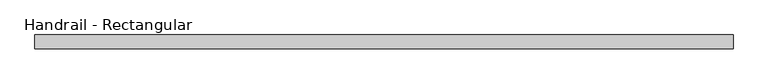
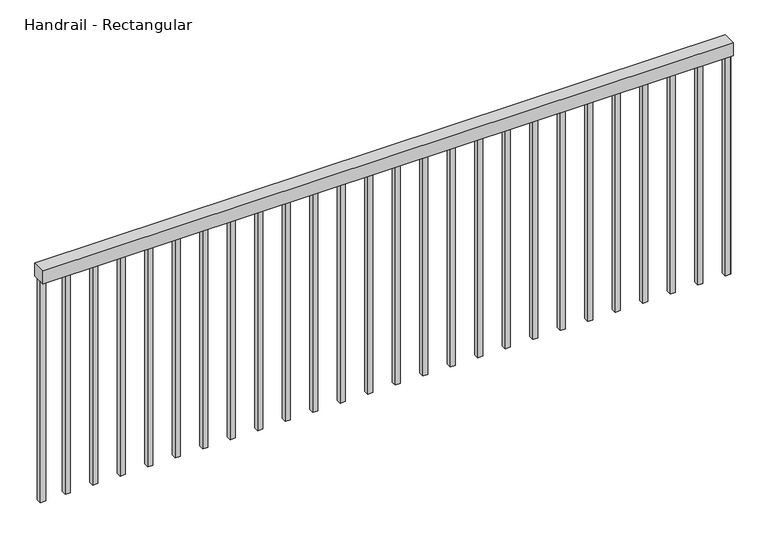
"""IFC4 building model written with IfcOpenShell, lengths in millimetres: railing geometry, Handrail - Rectangular."""

from ifc_helpers import new_model, si_unit, frame, origin, place, context, project, spatial, polyline, outline, extrude, source, transform, mapped, element, save


def handrail_rectangular_395b2247(model_context):
    return source(origin(), model_context, "Body", "SweptSolid", [
        extrude(outline(polyline([(-10635.2211091, 12195.0507146), (-10635.2211091, 12245.8507146), (-8085.2211091, 12245.8507146), (-8085.2211091, 12195.0507146), (-10635.2211091, 12195.0507146)])), frame((0.0, 0.0, 6654.4), z_axis=(0.0, 0.0, 1.0), x_axis=(1.0, 0.0, 0.0)), (0.0, 0.0, 1.0), 50.8),
        extrude(outline(polyline([(-8104.7461091, 12210.9257146), (-8104.7461091, 12229.9757146), (-8085.6961091, 12229.9757146), (-8085.6961091, 12210.9257146), (-8104.7461091, 12210.9257146)])), frame((0.0, 0.0, 5790.8), z_axis=(0.0, 0.0, 1.0), x_axis=(1.0, 0.0, 0.0)), (0.0, 0.0, 1.0), 863.6),
        extrude(outline(polyline([(-8206.3461091, 12210.9257146), (-8206.3461091, 12229.9757146), (-8187.2961091, 12229.9757146), (-8187.2961091, 12210.9257146), (-8206.3461091, 12210.9257146)])), frame((0.0, 0.0, 5790.8), z_axis=(0.0, 0.0, 1.0), x_axis=(1.0, 0.0, 0.0)), (0.0, 0.0, 1.0), 863.6),
        extrude(outline(polyline([(-8307.9461091, 12210.9257146), (-8307.9461091, 12229.9757146), (-8288.8961091, 12229.9757146), (-8288.8961091, 12210.9257146), (-8307.9461091, 12210.9257146)])), frame((0.0, 0.0, 5790.8), z_axis=(0.0, 0.0, 1.0), x_axis=(1.0, 0.0, 0.0)), (0.0, 0.0, 1.0), 863.6),
        extrude(outline(polyline([(-8409.5461091, 12210.9257146), (-8409.5461091, 12229.9757146), (-8390.4961091, 12229.9757146), (-8390.4961091, 12210.9257146), (-8409.5461091, 12210.9257146)])), frame((0.0, 0.0, 5790.8), z_axis=(0.0, 0.0, 1.0), x_axis=(1.0, 0.0, 0.0)), (0.0, 0.0, 1.0), 863.6),
        extrude(outline(polyline([(-8511.1461091, 12210.9257146), (-8511.1461091, 12229.9757146), (-8492.0961091, 12229.9757146), (-8492.0961091, 12210.9257146), (-8511.1461091, 12210.9257146)])), frame((0.0, 0.0, 5790.8), z_axis=(0.0, 0.0, 1.0), x_axis=(1.0, 0.0, 0.0)), (0.0, 0.0, 1.0), 863.6),
        extrude(outline(polyline([(-8612.7461091, 12210.9257146), (-8612.7461091, 12229.9757146), (-8593.6961091, 12229.9757146), (-8593.6961091, 12210.9257146), (-8612.7461091, 12210.9257146)])), frame((0.0, 0.0, 5790.8), z_axis=(0.0, 0.0, 1.0), x_axis=(1.0, 0.0, 0.0)), (0.0, 0.0, 1.0), 863.6),
        extrude(outline(polyline([(-8714.3461091, 12210.9257146), (-8714.3461091, 12229.9757146), (-8695.2961091, 12229.9757146), (-8695.2961091, 12210.9257146), (-8714.3461091, 12210.9257146)])), frame((0.0, 0.0, 5790.8), z_axis=(0.0, 0.0, 1.0), x_axis=(1.0, 0.0, 0.0)), (0.0, 0.0, 1.0), 863.6),
        extrude(outline(polyline([(-8815.9461091, 12210.9257146), (-8815.9461091, 12229.9757146), (-8796.8961091, 12229.9757146), (-8796.8961091, 12210.9257146), (-8815.9461091, 12210.9257146)])), frame((0.0, 0.0, 5790.8), z_axis=(0.0, 0.0, 1.0), x_axis=(1.0, 0.0, 0.0)), (0.0, 0.0, 1.0), 863.6),
        extrude(outline(polyline([(-8917.5461091, 12210.9257146), (-8917.5461091, 12229.9757146), (-8898.4961091, 12229.9757146), (-8898.4961091, 12210.9257146), (-8917.5461091, 12210.9257146)])), frame((0.0, 0.0, 5790.8), z_axis=(0.0, 0.0, 1.0), x_axis=(1.0, 0.0, 0.0)), (0.0, 0.0, 1.0), 863.6),
        extrude(outline(polyline([(-9019.1461091, 12210.9257146), (-9019.1461091, 12229.9757146), (-9000.0961091, 12229.9757146), (-9000.0961091, 12210.9257146), (-9019.1461091, 12210.9257146)])), frame((0.0, 0.0, 5790.8), z_axis=(0.0, 0.0, 1.0), x_axis=(1.0, 0.0, 0.0)), (0.0, 0.0, 1.0), 863.6),
        extrude(outline(polyline([(-9120.7461091, 12210.9257146), (-9120.7461091, 12229.9757146), (-9101.6961091, 12229.9757146), (-9101.6961091, 12210.9257146), (-9120.7461091, 12210.9257146)])), frame((0.0, 0.0, 5790.8), z_axis=(0.0, 0.0, 1.0), x_axis=(1.0, 0.0, 0.0)), (0.0, 0.0, 1.0), 863.6),
        extrude(outline(polyline([(-9222.3461091, 12210.9257146), (-9222.3461091, 12229.9757146), (-9203.2961091, 12229.9757146), (-9203.2961091, 12210.9257146), (-9222.3461091, 12210.9257146)])), frame((0.0, 0.0, 5790.8), z_axis=(0.0, 0.0, 1.0), x_axis=(1.0, 0.0, 0.0)), (0.0, 0.0, 1.0), 863.6),
        extrude(outline(polyline([(-9323.9461091, 12210.9257146), (-9323.9461091, 12229.9757146), (-9304.8961091, 12229.9757146), (-9304.8961091, 12210.9257146), (-9323.9461091, 12210.9257146)])), frame((0.0, 0.0, 5790.8), z_axis=(0.0, 0.0, 1.0), x_axis=(1.0, 0.0, 0.0)), (0.0, 0.0, 1.0), 863.6),
        extrude(outline(polyline([(-9425.5461091, 12210.9257146), (-9425.5461091, 12229.9757146), (-9406.4961091, 12229.9757146), (-9406.4961091, 12210.9257146), (-9425.5461091, 12210.9257146)])), frame((0.0, 0.0, 5790.8), z_axis=(0.0, 0.0, 1.0), x_axis=(1.0, 0.0, 0.0)), (0.0, 0.0, 1.0), 863.6),
        extrude(outline(polyline([(-9527.1461091, 12210.9257146), (-9527.1461091, 12229.9757146), (-9508.0961091, 12229.9757146), (-9508.0961091, 12210.9257146), (-9527.1461091, 12210.9257146)])), frame((0.0, 0.0, 5790.8), z_axis=(0.0, 0.0, 1.0), x_axis=(1.0, 0.0, 0.0)), (0.0, 0.0, 1.0), 863.6),
        extrude(outline(polyline([(-9628.7461091, 12210.9257146), (-9628.7461091, 12229.9757146), (-9609.6961091, 12229.9757146), (-9609.6961091, 12210.9257146), (-9628.7461091, 12210.9257146)])), frame((0.0, 0.0, 5790.8), z_axis=(0.0, 0.0, 1.0), x_axis=(1.0, 0.0, 0.0)), (0.0, 0.0, 1.0), 863.6),
        extrude(outline(polyline([(-9730.3461091, 12210.9257146), (-9730.3461091, 12229.9757146), (-9711.2961091, 12229.9757146), (-9711.2961091, 12210.9257146), (-9730.3461091, 12210.9257146)])), frame((0.0, 0.0, 5790.8), z_axis=(0.0, 0.0, 1.0), x_axis=(1.0, 0.0, 0.0)), (0.0, 0.0, 1.0), 863.6),
        extrude(outline(polyline([(-9831.9461091, 12210.9257146), (-9831.9461091, 12229.9757146), (-9812.8961091, 12229.9757146), (-9812.8961091, 12210.9257146), (-9831.9461091, 12210.9257146)])), frame((0.0, 0.0, 5790.8), z_axis=(0.0, 0.0, 1.0), x_axis=(1.0, 0.0, 0.0)), (0.0, 0.0, 1.0), 863.6),
        extrude(outline(polyline([(-9933.5461091, 12210.9257146), (-9933.5461091, 12229.9757146), (-9914.4961091, 12229.9757146), (-9914.4961091, 12210.9257146), (-9933.5461091, 12210.9257146)])), frame((0.0, 0.0, 5790.8), z_axis=(0.0, 0.0, 1.0), x_axis=(1.0, 0.0, 0.0)), (0.0, 0.0, 1.0), 863.6),
        extrude(outline(polyline([(-10035.1461091, 12210.9257146), (-10035.1461091, 12229.9757146), (-10016.0961091, 12229.9757146), (-10016.0961091, 12210.9257146), (-10035.1461091, 12210.9257146)])), frame((0.0, 0.0, 5790.8), z_axis=(0.0, 0.0, 1.0), x_axis=(1.0, 0.0, 0.0)), (0.0, 0.0, 1.0), 863.6),
        extrude(outline(polyline([(-10136.7461091, 12210.9257146), (-10136.7461091, 12229.9757146), (-10117.6961091, 12229.9757146), (-10117.6961091, 12210.9257146), (-10136.7461091, 12210.9257146)])), frame((0.0, 0.0, 5790.8), z_axis=(0.0, 0.0, 1.0), x_axis=(1.0, 0.0, 0.0)), (0.0, 0.0, 1.0), 863.6),
        extrude(outline(polyline([(-10238.3461091, 12210.9257146), (-10238.3461091, 12229.9757146), (-10219.2961091, 12229.9757146), (-10219.2961091, 12210.9257146), (-10238.3461091, 12210.9257146)])), frame((0.0, 0.0, 5790.8), z_axis=(0.0, 0.0, 1.0), x_axis=(1.0, 0.0, 0.0)), (0.0, 0.0, 1.0), 863.6),
        extrude(outline(polyline([(-10339.9461091, 12210.9257146), (-10339.9461091, 12229.9757146), (-10320.8961091, 12229.9757146), (-10320.8961091, 12210.9257146), (-10339.9461091, 12210.9257146)])), frame((0.0, 0.0, 5790.8), z_axis=(0.0, 0.0, 1.0), x_axis=(1.0, 0.0, 0.0)), (0.0, 0.0, 1.0), 863.6),
        extrude(outline(polyline([(-10441.5461091, 12210.9257146), (-10441.5461091, 12229.9757146), (-10422.4961091, 12229.9757146), (-10422.4961091, 12210.9257146), (-10441.5461091, 12210.9257146)])), frame((0.0, 0.0, 5790.8), z_axis=(0.0, 0.0, 1.0), x_axis=(1.0, 0.0, 0.0)), (0.0, 0.0, 1.0), 863.6),
        extrude(outline(polyline([(-10543.1461091, 12210.9257146), (-10543.1461091, 12229.9757146), (-10524.0961091, 12229.9757146), (-10524.0961091, 12210.9257146), (-10543.1461091, 12210.9257146)])), frame((0.0, 0.0, 5790.8), z_axis=(0.0, 0.0, 1.0), x_axis=(1.0, 0.0, 0.0)), (0.0, 0.0, 1.0), 863.6),
        extrude(outline(polyline([(-8104.2711091, 12210.9257146), (-8104.2711091, 12229.9757146), (-8085.2211091, 12229.9757146), (-8085.2211091, 12210.9257146), (-8104.2711091, 12210.9257146)])), frame((0.0, 0.0, 5790.8), z_axis=(0.0, 0.0, 1.0), x_axis=(1.0, 0.0, 0.0)), (0.0, 0.0, 1.0), 863.6),
        extrude(outline(polyline([(-10635.2211091, 12210.9257146), (-10635.2211091, 12229.9757146), (-10616.1711091, 12229.9757146), (-10616.1711091, 12210.9257146), (-10635.2211091, 12210.9257146)])), frame((0.0, 0.0, 5790.8), z_axis=(0.0, 0.0, 1.0), x_axis=(1.0, 0.0, 0.0)), (0.0, 0.0, 1.0), 863.6),
    ])


if __name__ == "__main__":
    model = new_model("IFC4")
    model_context = context("Model", 3, world=origin())
    ifc_project = project(units=[si_unit("LENGTHUNIT", "METRE", prefix="MILLI")], contexts=[model_context])
    site = spatial("IfcSite", under=ifc_project)
    building = spatial("IfcBuilding", under=site)
    placement = place(None, origin())
    handrail_rectangular_shape = handrail_rectangular_395b2247(model_context)
    element("IfcRailing", 1, ObjectType="Handrail - Rectangular", at=placement, inside=building, context=model_context, shape_type="MappedRepresentation", body=[
        mapped(handrail_rectangular_shape, transform((0.0, 0.0, 0.0), x_axis=(1.0, 0.0, 0.0), y_axis=(0.0, 1.0, 0.0), z_axis=(0.0, 0.0, 1.0))),
    ])
    save(model, "model.ifc")
